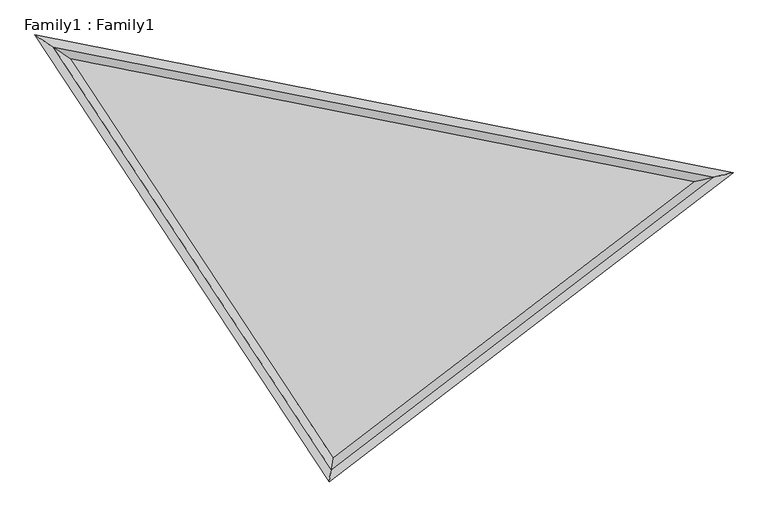
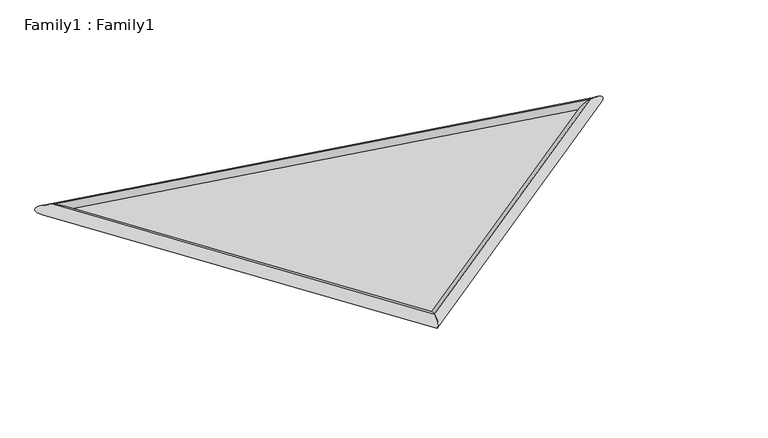
"""IFC4 building model written with IfcOpenShell, lengths in millimetres: proxy geometry, Family1 : Family1."""

from ifc_helpers import new_model, si_unit, frame, origin, origin_with_axes, place, context, project, spatial, polyline, ellipse_curve, outline, extrude, source, transform, mapped, element, save
from ifc_brep_helpers import cylinder_surface, advanced_brep


def family1_family1_cffea302(model_context):
    return source(origin(), model_context, "Body", "SolidModel", [
        extrude(outline(polyline([(515.0673386, -2339.1030023), (-2753.0542282, 2626.435907), (5004.9093406, 1096.6083001), (515.0673386, -2339.1030023)])), origin_with_axes(), (0.0, 0.0, 1.0), 34.1328789),
        advanced_brep(
        [(515.0673386, -2339.1030023, 100.0), (515.0673386, -2339.1030023, -100.0), (-2753.0542282, 2626.435907, -100.0), (-2753.0542282, 2626.435907, 100.0), (5004.9093406, 1096.6083001, -100.0), (5004.9093406, 1096.6083001, 100.0)],
        [
            (0, 1, ellipse_curve(frame((515.0673386, -2339.1030023, 0.0), z_axis=(-0.9859599620965575, 0.16698189465494423, 0.0), x_axis=(-0.16698189465494423, -0.9859599620965575, 0.0)), 146.7275817, 100.0)),
            (1, 2),
            (2, 3, ellipse_curve(frame((-2753.0542282, 2626.435907, 0.0), z_axis=(-0.5577737498328822, -0.8299930385234355, 0.0), x_axis=(0.8299930385234356, -0.5577737498328824, 0.0)), 258.6267019, 100.0)),
            (3, 0),
            (1, 0, ellipse_curve(frame((515.0673386, -2339.1030023, 0.0), z_axis=(-0.9859599620965575, 0.16698189465494423, 0.0), x_axis=(-0.16698189465494423, -0.9859599620965575, 0.0)), 146.7275817, 100.0)),
            (3, 2, ellipse_curve(frame((-2753.0542282, 2626.435907, 0.0), z_axis=(-0.5577737498328822, -0.8299930385234355, 0.0), x_axis=(0.8299930385234356, -0.5577737498328824, 0.0)), 258.6267019, 100.0)),
            (2, 4),
            (4, 5, ellipse_curve(frame((5004.9093406, 1096.6083001, 0.0), z_axis=(-0.2272343932855292, 0.9738400949376429, 0.0), x_axis=(-0.9738400949376429, -0.22723439328552913, 0.0)), 243.1027052, 100.0)),
            (5, 3),
            (5, 4, ellipse_curve(frame((5004.9093406, 1096.6083001, 0.0), z_axis=(-0.2272343932855292, 0.9738400949376429, 0.0), x_axis=(-0.9738400949376429, -0.22723439328552913, 0.0)), 243.1027052, 100.0)),
            (4, 1),
            (0, 5),
        ],
        [
            cylinder_surface(frame((515.0673386, -2339.1030023, 0.0), z_axis=(0.5497714273049605, -0.8353151367711869, 0.0), x_axis=(-0.8353151367711869, -0.5497714273049605, 0.0)), 100.0),
            cylinder_surface(frame((-2753.0542282, 2626.435907, 0.0), z_axis=(-0.9811064331513324, 0.19346877481668828, 0.0), x_axis=(0.19346877481668828, 0.9811064331513324, 0.0)), 100.0),
            cylinder_surface(frame((5004.9093406, 1096.6083001, 0.0), z_axis=(0.7941612544647704, 0.6077070856152185, 0.0), x_axis=(0.6077070856152185, -0.7941612544647704, 0.0)), 100.0),
        ],
        [
            (0, [[1, 2, 3, 4]]),
            (0, [[5, -4, 6, -2]]),
            (1, [[-3, 7, 8, 9]]),
            (1, [[-6, -9, 10, -7]]),
            (2, [[-8, 11, -1, 12]]),
            (2, [[-10, -12, -5, -11]]),
        ],
    ),
    ])


if __name__ == "__main__":
    model = new_model("IFC4")
    model_context = context("Model", 3, world=origin())
    ifc_project = project(units=[si_unit("LENGTHUNIT", "METRE", prefix="MILLI")], contexts=[model_context])
    site = spatial("IfcSite", under=ifc_project)
    building = spatial("IfcBuilding", under=site)
    placement = place(None, origin())
    family1_family1_shape = family1_family1_cffea302(model_context)
    element("IfcBuildingElementProxy", 1, Name="Family1 : Family1", ObjectType="Family1 : Family1", at=placement, inside=building, context=model_context, shape_type="MappedRepresentation", body=[
        mapped(family1_family1_shape, transform((0.0, 0.0, 0.0), x_axis=(1.0, 0.0, 0.0), y_axis=(0.0, 1.0, 0.0), z_axis=(0.0, 0.0, 1.0))),
    ])
    save(model, "model.ifc")

# Revit data of these elements
# Type "Family1 : Family1"
#   Default Elevation = 0
# Element 1 (IfcBuildingElementProxy, "Family1 : Family1")
#   Materials on its faces: "Glass"
# Materials
#   "Glass": class "Glass", colour RGB 0 128 192, transparency 0.9, Description = "Soda Lime Glass", Cost = 0
